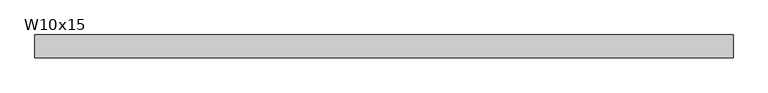
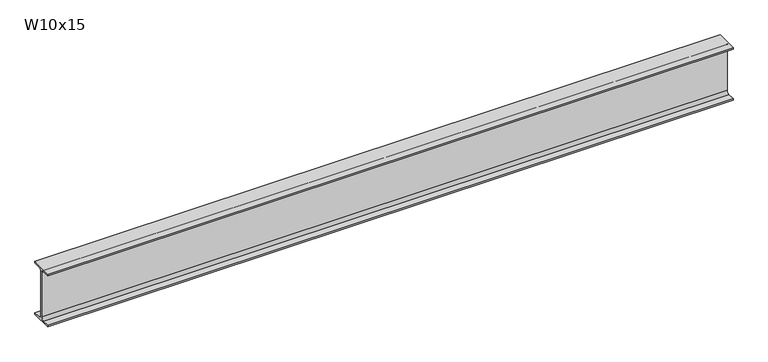
"""IFC4 building model written with IfcOpenShell, lengths in millimetres: beam geometry, RME W-Wide Flange : W10x15."""

from ifc_helpers import new_model, si_unit, point, frame, frame_2d, origin, place, context, project, spatial, polyline, circle_curve, trimmed, segment, composite_curve, outline, extrude, source, transform, mapped, element, save


def w10x15_f8958ef6(model_context):
    return source(origin(), model_context, "Body", "SweptSolid", [
        extrude(outline(composite_curve([segment(polyline([(50.8, -120.142), (50.8, -127.0), (-50.8, -127.0), (-50.8, -120.142), (-16.7005, -120.142)]), True, "CONTINUOUS"), segment(trimmed(circle_curve(frame_2d((-16.7005, -106.3625)), 13.7795), [point((-16.7005, -120.142))], [point((-2.921, -106.3625))], True, "CARTESIAN"), True, "CONTINUOUS"), segment(polyline([(-2.921, -106.3625), (-2.921, 106.3625)]), True, "CONTINUOUS"), segment(trimmed(circle_curve(frame_2d((-16.7005, 106.3625)), 13.7795), [point((-2.921, 106.3625))], [point((-16.7005, 120.142))], True, "CARTESIAN"), True, "CONTINUOUS"), segment(polyline([(-16.7005, 120.142), (-50.8, 120.142), (-50.8, 127.0), (50.8, 127.0), (50.8, 120.142), (16.7005, 120.142)]), True, "CONTINUOUS"), segment(trimmed(circle_curve(frame_2d((16.7005, 106.3625)), 13.7795), [point((16.7005, 120.142))], [point((2.921, 106.3625))], True, "CARTESIAN"), True, "CONTINUOUS"), segment(polyline([(2.921, 106.3625), (2.921, -106.3625)]), True, "CONTINUOUS"), segment(trimmed(circle_curve(frame_2d((16.7005, -106.3625)), 13.7795), [point((2.921, -106.3625))], [point((16.7005, -120.142))], True, "CARTESIAN"), True, "CONTINUOUS"), segment(polyline([(16.7005, -120.142), (50.8, -120.142)]), True, "CONTINUOUS")], self_intersect=False)), frame((-1562.7322907, 0.0, 0.0), z_axis=(1.0, 0.0, 0.0), x_axis=(0.0, 1.0, 0.0)), (0.0, 0.0, 1.0), 3125.4645815),
    ])


if __name__ == "__main__":
    model = new_model("IFC4")
    model_context = context("Model", 3, world=origin())
    ifc_project = project(units=[si_unit("LENGTHUNIT", "METRE", prefix="MILLI")], contexts=[model_context])
    site = spatial("IfcSite", under=ifc_project)
    building = spatial("IfcBuilding", under=site)
    placement = place(None, origin())
    w10x15_shape = w10x15_f8958ef6(model_context)
    element("IfcBeam", 1, ObjectType="RME W-Wide Flange : W10x15", at=placement, inside=building, context=model_context, shape_type="MappedRepresentation", body=[
        mapped(w10x15_shape, transform((0.0, 0.0, 0.0), x_axis=(1.0, 0.0, 0.0), y_axis=(0.0, 1.0, 0.0), z_axis=(0.0, 0.0, 1.0))),
    ])
    save(model, "model.ifc")

# Revit data of these elements
# Type "RME W-Wide Flange : W10x15"
#   WELD P [instance default] = ""
#   WELD LE [instance default] = ""
#   WELD D [instance default] = ""
#   TOP SECTION SIZE [instance default] = ""
#   TOP SECTION LENGTH [instance default] = ""
#   REMARKS [instance default] = ""
#   REINF TYPE [instance default] = ""
#   Nominal Size = "W24"
#   End Bearing Capacity [instance default] = ""
#   BOT SECTION SIZE [instance default] = ""
#   BOT SECTION LENGTH [instance default] = ""
#   Assembly Code = "B10"
#   W = 15
#   Start Extension Calculation [instance default] = 10' - 0"
#   Start Extension [instance default] = -0' - 0 1/2"
#   End Extension Calculation [instance default] = 10' - 0"
#   End Extension [instance default] = -0' - 0 1/2"
#   Length [instance default] = 5' - 0"
#   bf = 0' - 4"
#   d = 0' - 10"
#   k = 0' - 0 13/16"
#   k2 = 0' - 0.5425"
#   tf = 0' - 0.27"
#   tw = 0' - 0.23"
#   A = 0.030625 SF
#   Structural Material [instance default] = Metal - Steel - ASTM A992
# Element 1 (IfcBeam, "RME W-Wide Flange : W10x15")
#   Length = 10' - 3.04979"
#   Materials on its faces: "Metal - Steel - ASTM A992"
# Materials
#   "Metal - Steel - ASTM A992": class "Metal", colour RGB 255 128 0, transparency 0
